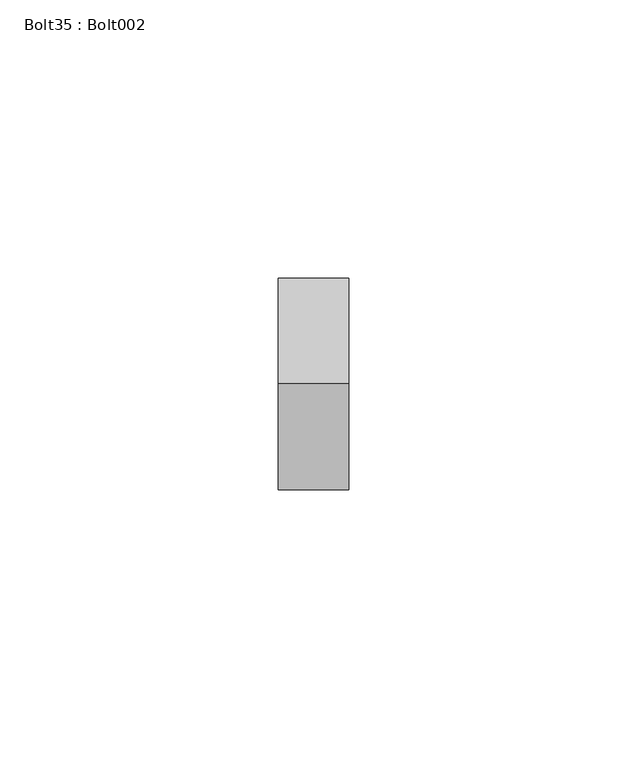
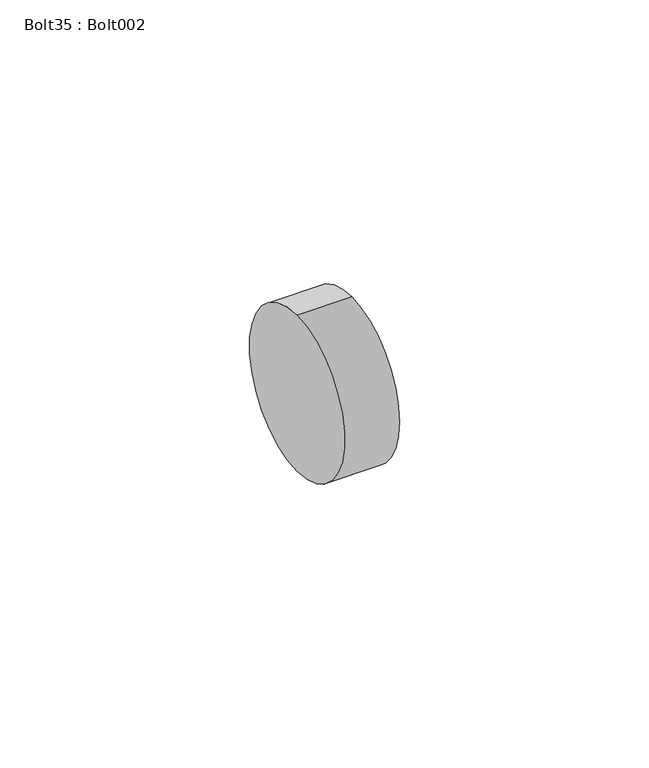
"""IFC4 building model written with IfcOpenShell, lengths in millimetres: proxy geometry, Bolt35 : Bolt002."""

from ifc_helpers import new_model, si_unit, point, frame, frame_2d, origin, place, context, project, spatial, circle_curve, trimmed, segment, composite_curve, outline, extrude, source, transform, mapped, element, save


def bolt35_bolt002_7273d207(model_context):
    return source(origin(), model_context, "Body", "SweptSolid", [
        extrude(outline(composite_curve([segment(trimmed(circle_curve(frame_2d((1896.5882072, 39960.0063132)), 19.05), [point((1896.5882072, 39979.0563132))], [point((1896.5882072, 39940.9563132))], False, "CARTESIAN"), True, "CONTINUOUS"), segment(trimmed(circle_curve(frame_2d((1896.5882072, 39960.0063132)), 19.05), [point((1896.5882072, 39940.9563132))], [point((1896.5882072, 39979.0563132))], False, "CARTESIAN"), True, "CONTINUOUS")], self_intersect=False)), frame((10268.2640809, 0.0, 0.0), z_axis=(1.0, 0.0, 0.0), x_axis=(0.0, 1.0, 0.0)), (0.0, 0.0, 1.0), 12.7),
    ])


if __name__ == "__main__":
    model = new_model("IFC4")
    model_context = context("Model", 3, world=origin())
    ifc_project = project(units=[si_unit("LENGTHUNIT", "METRE", prefix="MILLI")], contexts=[model_context])
    site = spatial("IfcSite", under=ifc_project)
    building = spatial("IfcBuilding", under=site)
    placement = place(None, origin())
    bolt35_bolt002_shape = bolt35_bolt002_7273d207(model_context)
    element("IfcBuildingElementProxy", 1, Name="Bolt35 : Bolt002", ObjectType="Bolt35 : Bolt002", at=placement, inside=building, context=model_context, shape_type="MappedRepresentation", body=[
        mapped(bolt35_bolt002_shape, transform((0.0, 0.0, 0.0), x_axis=(1.0, 0.0, 0.0), y_axis=(0.0, 1.0, 0.0), z_axis=(0.0, 0.0, 1.0))),
    ])
    save(model, "model.ifc")

# Revit data of these elements
# Type "Bolt35 : Bolt002"
#   NameOverride = "Bolt002"
# Element 1 (IfcBuildingElementProxy, "Bolt35 : Bolt002")
#   Materials on its faces: "STEEL ANGLE AND ANCHOR BOLT (SEE STRUCT. DWGS)"
# Materials
#   "STEEL ANGLE AND ANCHOR BOLT (SEE STRUCT. DWGS)": class "Unassigned", colour RGB 128 128 128, transparency 0, Cost = 0
